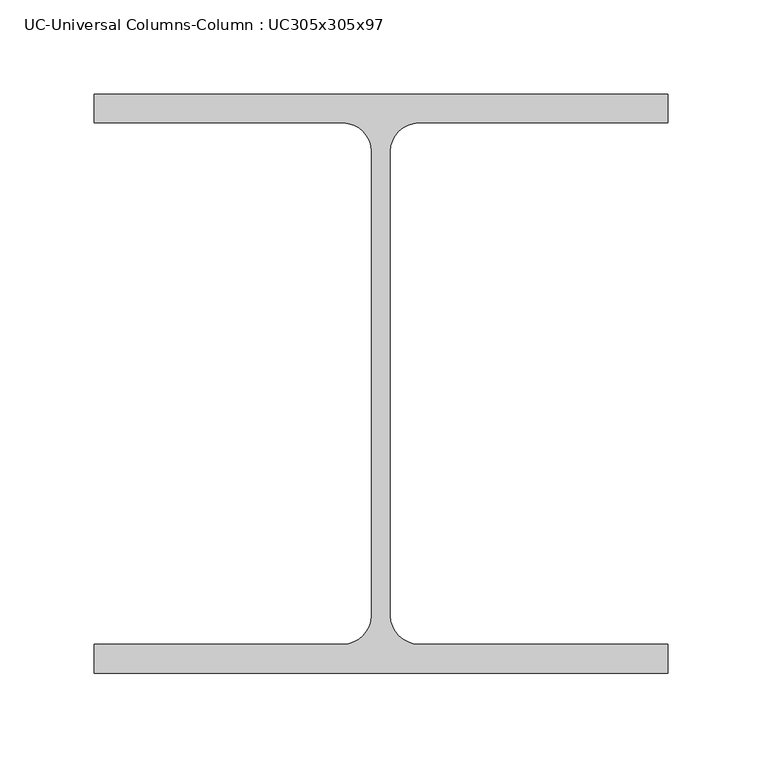
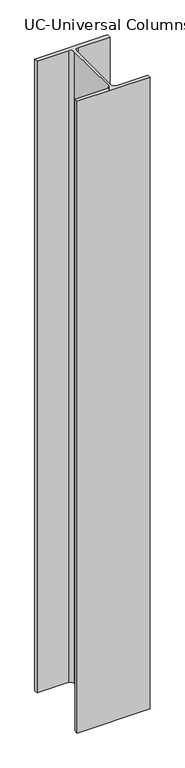
"""IFC4 building model written with IfcOpenShell, lengths in millimetres: column geometry, UC-Universal Columns-Column : UC305x305x97."""

from ifc_helpers import new_model, si_unit, point, frame, frame_2d, origin, place, context, project, spatial, polyline, circle_curve, trimmed, segment, composite_curve, outline, extrude, source, transform, mapped, element, save


def uc_universal_columns_column_uc305x305x97_6ea2ceb4(model_context):
    return source(origin(), model_context, "Body", "SweptSolid", [
        extrude(outline(composite_curve([segment(polyline([(152.65, 153.95), (152.65, 138.55), (20.15, 138.55)]), True, "CONTINUOUS"), segment(trimmed(circle_curve(frame_2d((20.15, 123.35)), 15.2), [point((20.15, 138.55))], [point((4.95, 123.35))], True, "CARTESIAN"), True, "CONTINUOUS"), segment(polyline([(4.95, 123.35), (4.95, -123.35)]), True, "CONTINUOUS"), segment(trimmed(circle_curve(frame_2d((20.15, -123.35)), 15.2), [point((4.95, -123.35))], [point((20.15, -138.55))], True, "CARTESIAN"), True, "CONTINUOUS"), segment(polyline([(20.15, -138.55), (152.65, -138.55), (152.65, -153.95), (-152.65, -153.95), (-152.65, -138.55), (-20.15, -138.55)]), True, "CONTINUOUS"), segment(trimmed(circle_curve(frame_2d((-20.15, -123.35)), 15.2), [point((-20.15, -138.55))], [point((-4.95, -123.35))], True, "CARTESIAN"), True, "CONTINUOUS"), segment(polyline([(-4.95, -123.35), (-4.95, 123.35)]), True, "CONTINUOUS"), segment(trimmed(circle_curve(frame_2d((-20.15, 123.35)), 15.2), [point((-4.95, 123.35))], [point((-20.15, 138.55))], True, "CARTESIAN"), True, "CONTINUOUS"), segment(polyline([(-20.15, 138.55), (-152.65, 138.55), (-152.65, 153.95), (152.65, 153.95)]), True, "CONTINUOUS")], self_intersect=False)), frame((0.0, 0.0, -594.0), z_axis=(0.0, 0.0, 1.0), x_axis=(1.0, 0.0, 0.0)), (0.0, 0.0, 1.0), 2793.0),
    ])


if __name__ == "__main__":
    model = new_model("IFC4")
    model_context = context("Model", 3, world=origin())
    ifc_project = project(units=[si_unit("LENGTHUNIT", "METRE", prefix="MILLI")], contexts=[model_context])
    site = spatial("IfcSite", under=ifc_project)
    building = spatial("IfcBuilding", under=site)
    placement = place(None, origin())
    uc_universal_columns_column_uc305x305x97_shape = uc_universal_columns_column_uc305x305x97_6ea2ceb4(model_context)
    element("IfcColumn", 1, ObjectType="UC-Universal Columns-Column : UC305x305x97", at=placement, inside=building, context=model_context, shape_type="MappedRepresentation", body=[
        mapped(uc_universal_columns_column_uc305x305x97_shape, transform((0.0, 0.0, 0.0), x_axis=(1.0, 0.0, 0.0), y_axis=(0.0, 1.0, 0.0), z_axis=(0.0, 0.0, 1.0))),
    ])
    save(model, "model.ifc")

# Revit data of these elements
# Project information
#   Project Issue Date = "Issue Date"
#   Project Status = "Project Status"
#   Client Name = "Owner"
#   Project Address = "Enter address here"
#   Project Name = "Project Name"
#   Project Number = "0001"
# Type "UC-Universal Columns-Column : UC305x305x97"
#   Section Name Key = "UC305x305x97"
#   Cost = 5
#   Width = 30.53 cm
#   Web Thickness = 0.99 cm
#   Web Fillet = 1.52 cm
#   Warping Constant = 1560000.0 cm⁶
#   Torsional Moment of Inertia = 91.20 cm⁴
#   Section Area = 123.0 cm²
#   Plastic Modulus weak axis = 726.0 cm³
#   Plastic Modulus strong axis = 1592.0 cm³
#   Nominal Weight = 96.8996 kgf/m
#   Moment of Inertia weak axis = 7308.00 cm⁴
#   Moment of Inertia strong axis = 22249.00 cm⁴
#   Height = 30.79 cm
#   Flange Thickness = 1.54 cm
#   Elastic Modulus weak axis = 479.0 cm³
#   Elastic Modulus strong axis = 1445.0 cm³
#   Centroid Vertical = 15.395 cm
#   Centroid Horizontal = 15.265 cm
#   Bolt Spacing = 14.0 cm
#   Structural Material [instance default] = Metal - Steel 43-275
#   Type Comments = ""
#   Assembly Code = ""
# Element 1 (IfcColumn, "UC-Universal Columns-Column : UC305x305x97")
#   Materials on its faces: "Metal - Steel 43-275"
# Materials
#   "Metal - Steel 43-275": class "Metal", colour RGB 247 247 247, transparency 0, Cost = 0
